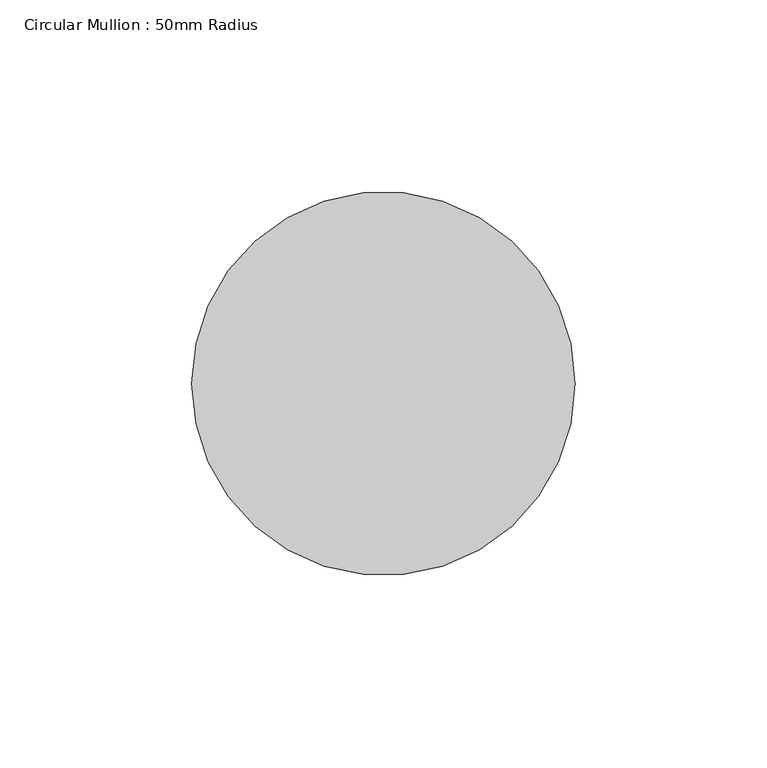
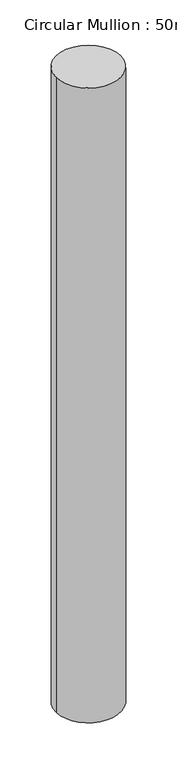
"""IFC4 building model written with IfcOpenShell, lengths in millimetres: member geometry, Circular Mullion : 50mm Radius."""

from ifc_helpers import new_model, si_unit, point, frame, origin, origin_2d, place, context, project, spatial, circle_curve, trimmed, segment, composite_curve, outline, extrude, source, transform, mapped, element, save


def circular_mullion_50mm_radius_ec9e6593(model_context):
    return source(origin(), model_context, "Body", "SweptSolid", [
        extrude(outline(composite_curve([segment(trimmed(circle_curve(origin_2d(), 50.0), [point((50.0, 0.0))], [point((-50.0, 0.0))], False, "CARTESIAN"), True, "CONTINUOUS"), segment(trimmed(circle_curve(origin_2d(), 50.0), [point((-50.0, 0.0))], [point((50.0, 0.0))], False, "CARTESIAN"), True, "CONTINUOUS")], self_intersect=False)), frame((0.0, 0.0, -1037.72619), z_axis=(0.0, 0.0, 1.0), x_axis=(1.0, 0.0, 0.0)), (0.0, 0.0, 1.0), 1037.72619),
    ])


if __name__ == "__main__":
    model = new_model("IFC4")
    model_context = context("Model", 3, world=origin())
    ifc_project = project(units=[si_unit("LENGTHUNIT", "METRE", prefix="MILLI")], contexts=[model_context])
    site = spatial("IfcSite", under=ifc_project)
    building = spatial("IfcBuilding", under=site)
    placement = place(None, origin())
    circular_mullion_50mm_radius_shape = circular_mullion_50mm_radius_ec9e6593(model_context)
    element("IfcMember", 1, ObjectType="Circular Mullion : 50mm Radius", at=placement, inside=building, context=model_context, shape_type="MappedRepresentation", body=[
        mapped(circular_mullion_50mm_radius_shape, transform((0.0, 0.0, 0.0), x_axis=(1.0, 0.0, 0.0), y_axis=(0.0, 1.0, 0.0), z_axis=(0.0, 0.0, 1.0))),
    ])
    save(model, "model.ifc")

# Revit data of these elements
# Type "Circular Mullion : 50mm Radius"
#   built-in parameter 1007350 = 0.164042 (stored number, unit not read)
# Element 1 (IfcMember, "Circular Mullion : 50mm Radius")
#   Materials on its faces: "Aluminium"
# Materials
#   "Aluminium": class "Metal", colour RGB 247 247 247, transparency 0, Description = "Aluminium 6061", Cost = 0
